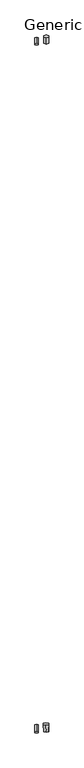
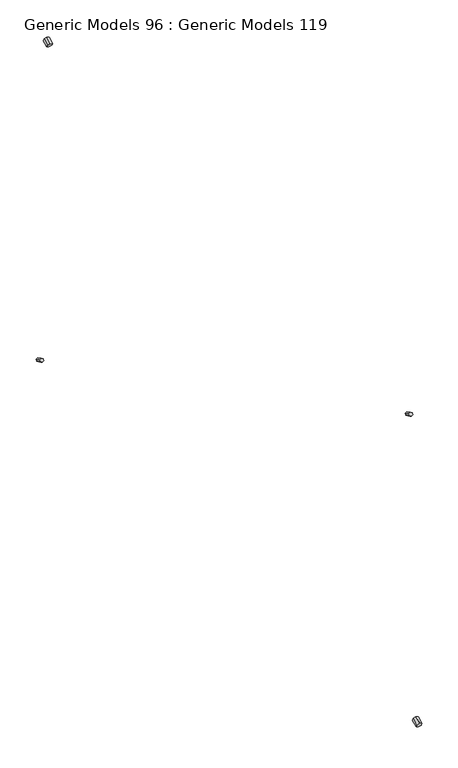
"""IFC4 building model written with IfcOpenShell, lengths in millimetres: proxy geometry, Generic Models 96 : Generic Models 119."""

from ifc_helpers import new_model, si_unit, frame, origin, place, context, project, spatial, polyline, outline, extrude, faceted_brep, source, transform, mapped, element, save


def generic_models_96_generic_models_119_cda3f510(model_context):
    return source(origin(), model_context, "Body", "SolidModel", [
        faceted_brep([(31987.4987939, 30893.1483324, 266471.7687657), (31987.4987939, 30901.8757314, 266454.8355142), (32003.9965778, 30906.2394309, 266446.3688884), (32020.4943618, 30901.8757314, 266454.8355142), (32020.4943618, 30893.1483324, 266471.7687657), (32003.9965778, 30888.7846329, 266480.2353914), (31985.9472947, 30934.9577151, 266493.3173244), (32002.4450787, 30930.5940156, 266501.7839502), (32018.9428626, 30934.9577151, 266493.3173244), (32018.9428626, 30943.6851141, 266476.3840729), (32002.4450787, 30948.0488136, 266467.9174471), (31985.9472947, 30943.6851141, 266476.3840729)], [[[0, 1, 2, 3, 4, 5]], [[6, 7, 8, 9, 10, 11]], [[6, 11, 1, 0]], [[11, 10, 2, 1]], [[10, 9, 3, 2]], [[9, 8, 4, 3]], [[8, 7, 5, 4]], [[7, 6, 0, 5]]]),
        faceted_brep([(31956.3469127, 30934.4369056, 268642.8051671), (31956.3469127, 30928.6029373, 268631.5244396), (31945.3483901, 30925.6859532, 268625.8840758), (31934.3498675, 30928.6029373, 268631.5244396), (31934.3498675, 30934.4369056, 268642.8051671), (31945.3483901, 30937.3538897, 268648.4455309), (31956.2923001, 30892.5813314, 268664.4512968), (31945.2937775, 30895.4983155, 268670.0916606), (31934.2952549, 30892.5813314, 268664.4512968), (31934.2952549, 30886.7473631, 268653.1705692), (31945.2937775, 30883.830379, 268647.5302054), (31956.2923001, 30886.7473631, 268653.1705692)], [[[0, 1, 2, 3, 4, 5]], [[6, 7, 8, 9, 10, 11]], [[6, 11, 1, 0]], [[11, 10, 2, 1]], [[10, 9, 3, 2]], [[9, 8, 4, 3]], [[8, 7, 5, 4]], [[7, 6, 0, 5]]]),
        extrude(outline(polyline([(-9.525, 16.4977839), (9.5249999, 16.4977839), (19.0499999, 0.0), (9.5249999, -16.497784), (-9.525, -16.497784), (-19.0500001, 0.0), (-9.525, 16.4977839)])), frame((32003.9965778, 35128.3976646, 268644.0035888), z_axis=(0.0, 0.8888845937971597, 0.45813118089697674), x_axis=(0.0, 0.45813118089697674, -0.8888845937971597)), (0.0, 0.0, 1.0), 44.45),
        faceted_brep([(31956.3469127, 35161.0252375, 266456.9170821), (31956.3469127, 35155.1912692, 266445.6363545), (31945.3483901, 35152.2742851, 266439.9959907), (31934.3498675, 35155.1912692, 266445.6363545), (31934.3498675, 35161.0252375, 266456.9170821), (31945.3483901, 35163.9422216, 266462.5574459), (31956.2923001, 35121.542691, 266477.335971), (31945.2937775, 35124.4596751, 266482.9763347), (31934.2952549, 35121.542691, 266477.335971), (31934.2952549, 35115.7087227, 266466.0552434), (31945.2937775, 35112.7917386, 266460.4148796), (31956.2923001, 35115.7087227, 266466.0552434)], [[[0, 1, 2, 3, 4, 5]], [[6, 7, 8, 9, 10, 11]], [[6, 11, 1, 0]], [[11, 10, 2, 1]], [[10, 9, 3, 2]], [[9, 8, 4, 3]], [[8, 7, 5, 4]], [[7, 6, 0, 5]]]),
    ])


if __name__ == "__main__":
    model = new_model("IFC4")
    model_context = context("Model", 3, world=origin())
    ifc_project = project(units=[si_unit("LENGTHUNIT", "METRE", prefix="MILLI")], contexts=[model_context])
    site = spatial("IfcSite", under=ifc_project)
    building = spatial("IfcBuilding", under=site)
    placement = place(None, origin())
    generic_models_96_generic_models_119_shape = generic_models_96_generic_models_119_cda3f510(model_context)
    element("IfcBuildingElementProxy", 1, Name="Generic Models 96 : Generic Models 119", ObjectType="Generic Models 96 : Generic Models 119", at=placement, inside=building, context=model_context, shape_type="MappedRepresentation", body=[
        mapped(generic_models_96_generic_models_119_shape, transform((0.0, 0.0, 0.0), x_axis=(1.0, 0.0, 0.0), y_axis=(0.0, 1.0, 0.0), z_axis=(0.0, 0.0, 1.0))),
    ])
    save(model, "model.ifc")
